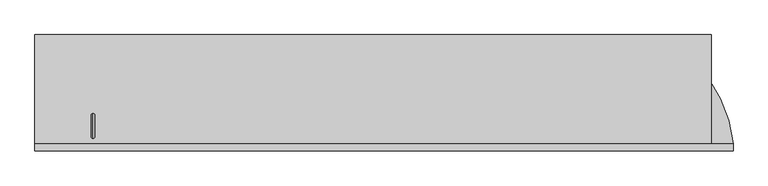
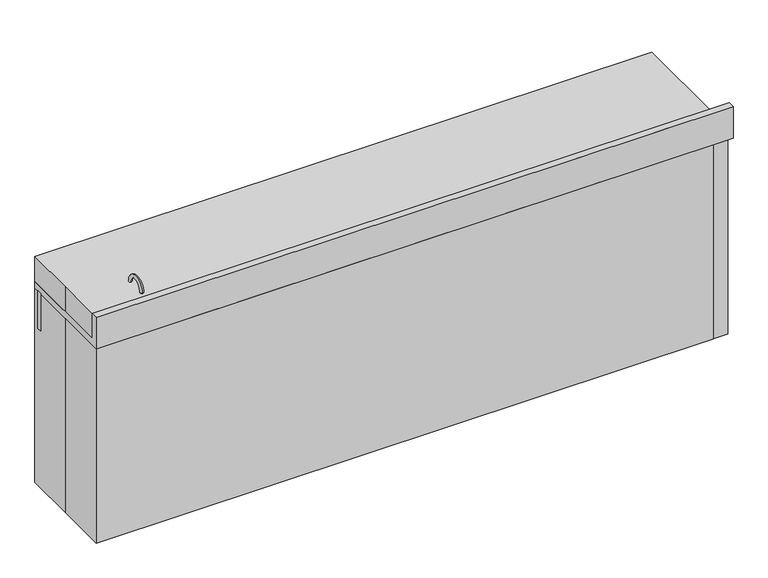
"""IFC4 building model written with IfcOpenShell, lengths in millimetres: proxy geometry, D0680 - Console, Accessory-Side, Dental Operatory-south sink-rounded : U0026 - Cabinet, Dental, Doctor's, Prosthodontic 2."""

import ifcopenshell
import ifcopenshell.guid

model = None  # the IFC model being written
_history = None  # IfcOwnerHistory: only IFC2X3 demands one
_inside = {}  # id of a spatial element -> (the spatial element, [elements in it])
_under = {}  # id of a project, library or spatial element -> (it, [spatial elements below it])
_declared = {}  # id of a project -> (the project, [libraries it declares])
_typed = {}  # id of a type object -> (the type object, [elements of that type])
_made_of = {}  # id of a material, layer set ... -> (it, [elements and type objects made of it])


def new_model(schema):
    """Start an empty IFC model of exactly this schema.

    Asked for "IFC4X3", IfcOpenShell would pick the latest addendum, in which some entities
    have other attributes; the version numbers below select the first issue.
    IFC2X3 requires an IfcOwnerHistory on every rooted entity: one is made here for all.
    """
    global model, _history
    if schema == "IFC4X3":
        model = ifcopenshell.file(schema_version=(4, 3, 0, 0))
    else:
        model = ifcopenshell.file(schema=schema)
    _inside.clear()
    _under.clear()
    _declared.clear()
    _typed.clear()
    _made_of.clear()
    _history = None
    if model.schema == "IFC2X3":
        org = make("IfcOrganization", Name="unknown")
        user = make(
            "IfcPersonAndOrganization",
            ThePerson=make("IfcPerson", FamilyName="unknown"),
            TheOrganization=org,
        )
        app = make(
            "IfcApplication",
            ApplicationDeveloper=org,
            Version="unknown",
            ApplicationFullName="unknown",
            ApplicationIdentifier="unknown",
        )
        _history = make(
            "IfcOwnerHistory",
            OwningUser=user,
            OwningApplication=app,
            ChangeAction="ADDED",
            CreationDate=0,
        )
    return model


def make(cls, **values):
    """One entity of the class cls with the attributes given. An attribute that is None is left unset."""
    return model.create_entity(
        cls, **{name: value for name, value in values.items() if value is not None}
    )


def rooted(cls, **values):
    """An entity with a GlobalId (a new one), such as an element, a storey or a relation."""
    return make(cls, GlobalId=ifcopenshell.guid.new(), OwnerHistory=_history, **values)


def si_unit(unit_type, name, prefix=None):
    """IfcSIUnit, for example si_unit("LENGTHUNIT", "METRE", prefix="MILLI")."""
    return make("IfcSIUnit", UnitType=unit_type, Prefix=prefix, Name=name)


def assignment(units):
    """IfcUnitAssignment: the units of a project."""
    return None if units is None else make("IfcUnitAssignment", Units=units)


def point(xyz):
    """IfcCartesianPoint."""
    return None if xyz is None else make("IfcCartesianPoint", Coordinates=xyz)


def direction(xyz):
    """IfcDirection."""
    return None if xyz is None else make("IfcDirection", DirectionRatios=xyz)


def frame(location, z_axis=None, x_axis=None):
    """IfcAxis2Placement3D, a coordinate frame: its origin and axes. An axis left out is left unset."""
    return make(
        "IfcAxis2Placement3D",
        Location=point(location),
        Axis=direction(z_axis),
        RefDirection=direction(x_axis),
    )


def frame_2d(location, x_axis=None):
    """IfcAxis2Placement2D, a coordinate frame in the plane: its origin and x axis."""
    return make(
        "IfcAxis2Placement2D", Location=point(location), RefDirection=direction(x_axis)
    )


def origin():
    """The frame at (0, 0, 0) with its axes left unset."""
    return frame((0.0, 0.0, 0.0))


def origin_with_axes():
    """The frame at (0, 0, 0) with the z axis (0, 0, 1) and the x axis (1, 0, 0) written out."""
    return frame((0.0, 0.0, 0.0), z_axis=(0.0, 0.0, 1.0), x_axis=(1.0, 0.0, 0.0))


def place(relative_to, where):
    """IfcLocalPlacement: puts the frame where relative to a parent placement (None: the world)."""
    return make(
        "IfcLocalPlacement", PlacementRelTo=relative_to, RelativePlacement=where
    )


def context(
    kind, dimensions, precision=None, world=None, true_north=None, identifier=None
):
    """IfcGeometricRepresentationContext, for example the 3D "Model" context."""
    return make(
        "IfcGeometricRepresentationContext",
        ContextIdentifier=identifier,
        ContextType=kind,
        CoordinateSpaceDimension=dimensions,
        Precision=precision,
        WorldCoordinateSystem=world,
        TrueNorth=true_north,
    )


def project(units=None, contexts=None):
    """IfcProject with its units and contexts."""
    return rooted(
        "IfcProject",
        Name="project",
        RepresentationContexts=contexts,
        UnitsInContext=assignment(units),
    )


def spatial(cls, under=None, at=None, **own):
    """A site, building, storey or space (cls), placed at a placement, below another one or the project."""
    s = rooted(cls, ObjectPlacement=at, **own)
    if under is not None:
        _under.setdefault(under.id(), (under, []))[1].append(s)
    return s


def polyline(points):
    """IfcPolyline through the points."""
    return make("IfcPolyline", Points=[point(p) for p in points])


def circle_curve(where, radius):
    """IfcCircle in the frame where."""
    return make("IfcCircle", Position=where, Radius=radius)


def ellipse_curve(where, semi_axis1, semi_axis2):
    """IfcEllipse in the frame where."""
    return make(
        "IfcEllipse", Position=where, SemiAxis1=semi_axis1, SemiAxis2=semi_axis2
    )


def trimmed(basis, trim1, trim2, sense, master):
    """IfcTrimmedCurve: the piece of a basis curve between two trims."""
    return make(
        "IfcTrimmedCurve",
        BasisCurve=basis,
        Trim1=trim1,
        Trim2=trim2,
        SenseAgreement=sense,
        MasterRepresentation=master,
    )


def segment(curve, same_sense, transition):
    """IfcCompositeCurveSegment."""
    return make(
        "IfcCompositeCurveSegment",
        Transition=transition,
        SameSense=same_sense,
        ParentCurve=curve,
    )


def composite_curve(segments, self_intersect=None):
    """IfcCompositeCurve: segments joined end to end."""
    return make("IfcCompositeCurve", Segments=segments, SelfIntersect=self_intersect)


def outline(outer, holes=None, kind="AREA"):
    """IfcArbitraryClosedProfileDef: a profile drawn as a closed curve; with holes, ...WithVoids."""
    if holes is None:
        return make("IfcArbitraryClosedProfileDef", ProfileType=kind, OuterCurve=outer)
    return make(
        "IfcArbitraryProfileDefWithVoids",
        ProfileType=kind,
        OuterCurve=outer,
        InnerCurves=holes,
    )


def extrude(swept, where, along, depth):
    """IfcExtrudedAreaSolid: the profile swept, set in the frame where, extruded along a direction by depth."""
    return make(
        "IfcExtrudedAreaSolid",
        SweptArea=swept,
        Position=where,
        ExtrudedDirection=direction(along),
        Depth=depth,
    )


def shape(context_of_items, identifier, shape_type, items):
    """IfcShapeRepresentation: the items that make up one representation, for example the "Body"."""
    return make(
        "IfcShapeRepresentation",
        ContextOfItems=context_of_items,
        RepresentationIdentifier=identifier,
        RepresentationType=shape_type,
        Items=items,
    )


def source(mapping_origin, context_of_items, identifier, shape_type, items):
    """IfcRepresentationMap: a shape defined once, which mapped items show again and again."""
    return make(
        "IfcRepresentationMap",
        MappingOrigin=mapping_origin,
        MappedRepresentation=shape(context_of_items, identifier, shape_type, items),
    )


def transform(
    local_origin,
    x_axis=None,
    y_axis=None,
    z_axis=None,
    scale=None,
    scale2=None,
    scale3=None,
    uniform=True,
):
    """IfcCartesianTransformationOperator3D, or its non-uniform kind. x_axis, y_axis, z_axis: its Axis1, 2, 3."""
    if uniform:
        return make(
            "IfcCartesianTransformationOperator3D",
            Axis1=direction(x_axis),
            Axis2=direction(y_axis),
            LocalOrigin=point(local_origin),
            Scale=scale,
            Axis3=direction(z_axis),
        )
    return make(
        "IfcCartesianTransformationOperator3DnonUniform",
        Axis1=direction(x_axis),
        Axis2=direction(y_axis),
        LocalOrigin=point(local_origin),
        Scale=scale,
        Axis3=direction(z_axis),
        Scale2=scale2,
        Scale3=scale3,
    )


def mapped(mapping_source, mapping_target):
    """IfcMappedItem: shows the shape of a source again, moved by a transform."""
    return make(
        "IfcMappedItem", MappingSource=mapping_source, MappingTarget=mapping_target
    )


def made_of(thing, what):
    """Note that an element or type object is made of a material, layer set ...; save() writes the relation."""
    if what is not None:
        _made_of.setdefault(what.id(), (what, []))[1].append(thing)
    return thing


def element(
    cls,
    number,
    at=None,
    inside=None,
    cuts=None,
    type_object=None,
    material=None,
    context=None,
    identifier="Body",
    shape_type=None,
    held_by="IfcProductDefinitionShape",
    body=None,
    shapes=None,
    **own,
):
    """One element of the class cls, such as IfcWall. Its Tag is "e" and its number.

    at: its placement. inside: the storey or other place that contains it. cuts: it is an
    opening in that element (IfcRelVoidsElement). A single representation is given by context,
    identifier, shape_type and body (its items); several are given by shapes. held_by: the class
    of the entity that holds the representations. save() writes the other relations.
    """
    e = rooted(cls, Tag="e%d" % number, ObjectPlacement=at, **own)
    if body is not None:
        shapes = [shape(context, identifier, shape_type, body)]
    if shapes is not None:
        e.Representation = make(held_by, Representations=shapes)
    if inside is not None:
        _inside.setdefault(inside.id(), (inside, []))[1].append(e)
    if cuts is not None:
        rooted(
            "IfcRelVoidsElement", RelatingBuildingElement=cuts, RelatedOpeningElement=e
        )
    if type_object is not None:
        _typed.setdefault(type_object.id(), (type_object, []))[1].append(e)
    return made_of(e, material)


def aggregate(whole, parts):
    """IfcRelAggregates: a whole, such as a stair, and the parts it consists of."""
    return rooted("IfcRelAggregates", RelatingObject=whole, RelatedObjects=parts)


def save(model, path):
    """Write the relations noted so far, then the file.

    IfcRelAggregates (storeys below a building ...), IfcRelContainedInSpatialStructure (elements
    in a storey), IfcRelDefinesByType, IfcRelAssociatesMaterial and IfcRelDeclares: one each for
    every whole, place, type object, material and project.
    """
    for whole, parts in _under.values():
        aggregate(whole, parts)
    for where, things in _inside.values():
        rooted(
            "IfcRelContainedInSpatialStructure",
            RelatedElements=things,
            RelatingStructure=where,
        )
    for kind, things in _typed.values():
        rooted("IfcRelDefinesByType", RelatedObjects=things, RelatingType=kind)
    for what, things in _made_of.values():
        rooted("IfcRelAssociatesMaterial", RelatedObjects=things, RelatingMaterial=what)
    for by, libraries in _declared.values():
        rooted("IfcRelDeclares", RelatingContext=by, RelatedDefinitions=libraries)
    model.write(path)


def plane_surface(at):
    """IfcPlane: the flat surface through the origin of the frame at, square to its z axis."""
    return make("IfcPlane", Position=at)


def cylinder_surface(at, radius):
    """IfcCylindricalSurface: all points at the distance radius from the z axis of the frame at."""
    return make("IfcCylindricalSurface", Position=at, Radius=radius)


def revolved_surface(curve, axis_point, axis_direction):
    """IfcSurfaceOfRevolution: the curve turned about the line through axis_point along axis_direction."""
    return make(
        "IfcSurfaceOfRevolution",
        SweptCurve=make("IfcArbitraryOpenProfileDef", ProfileType="CURVE", Curve=curve),
        AxisPosition=make("IfcAxis1Placement", Location=point(axis_point), Axis=direction(axis_direction)),
    )


def advanced_brep(points, edges, surfaces, faces):
    """IfcAdvancedBrep: a solid bounded by faces that lie on surfaces and meet in shared edges.

    An edge is (start, end): straight between two places in points (the first is 0);
    or (start, end, curve); or (start, end, curve, False) where it runs against its curve.
    A face is (place in surfaces, loops), or (place, loops, False) where it looks against
    its surface's normal. A loop lists edges by number (the first is 1), with a minus sign
    where the edge is run from its end to its start. The first loop is the outer one.
    """
    corners = [point(p) for p in points]
    vertices = [make("IfcVertexPoint", VertexGeometry=c) for c in corners]
    made = []
    for start, end, *more in edges:
        made.append(
            make(
                "IfcEdgeCurve",
                EdgeStart=vertices[start],
                EdgeEnd=vertices[end],
                EdgeGeometry=more[0] if more else make("IfcPolyline", Points=[corners[start], corners[end]]),
                SameSense=more[1] if len(more) > 1 else True,
            )
        )
    hull = []
    for where, loops, *sense in faces:
        bounds = []
        for j, loop in enumerate(loops):
            ring = [make("IfcOrientedEdge", EdgeElement=made[abs(k) - 1], Orientation=k > 0) for k in loop]
            bounds.append(
                make(
                    "IfcFaceOuterBound" if j == 0 else "IfcFaceBound",
                    Bound=make("IfcEdgeLoop", EdgeList=ring),
                    Orientation=True,
                )
            )
        hull.append(make("IfcAdvancedFace", Bounds=bounds, FaceSurface=surfaces[where], SameSense=sense[0] if sense else True))
    return make("IfcAdvancedBrep", Outer=make("IfcClosedShell", CfsFaces=hull))


def specialty_equipment_bc5c30ac(model_context):
    return source(origin(), model_context, "Body", "SolidModel", [
        advanced_brep(
        [(-1014.0443585, 165.0080446, 787.3899582), (-1014.0443585, 153.8955446, 787.3899582), (-1014.0443585, -128.6794554, 787.3899582), (-1014.0443585, -139.7919554, 787.3899582), (-1014.0443585, 152.3080446, 785.8024582), (-1014.0443585, -127.0919554, 785.8024582), (-1014.0443585, 152.3080446, 730.25), (-1014.0443585, -127.0919554, 730.25), (-1014.0443585, 101.5080446, 679.45), (-1014.0443585, 25.2053012, 679.45), (-1003.5461263, 12.6976148, 679.45), (-1014.0443585, 0.1899284, 679.45), (-1014.0443585, -76.2919554, 679.45), (-1028.9461263, 12.6976148, 679.45), (-1014.0443585, 158.6580446, 676.275), (-1014.0443585, 158.6580446, 784.0168572), (-1014.0443585, -133.4419554, 784.0168572), (-1014.0443585, -133.4419554, 676.275), (-1014.0443585, 165.0080446, 784.0168572), (-1014.0443585, -139.7919554, 784.0168572), (-1014.0443585, 0.1899284, 676.275), (-1003.5461263, 12.6976148, 676.275), (-1014.0443585, 25.2053012, 676.275), (-1028.9461263, 12.6976148, 676.275)],
        [
            (0, 1),
            (1, 2, circle_curve(frame((-1014.0443585, 12.6080446, 787.3899582), z_axis=(0.0, 0.0, -1.0), x_axis=(0.0, -1.0, 0.0)), 141.2875)),
            (2, 3),
            (3, 0, circle_curve(frame((-1014.0443585, 12.6080446, 787.3899582), z_axis=(0.0, 0.0, 1.0), x_axis=(0.0, -1.0, 0.0)), 152.4)),
            (2, 1, circle_curve(frame((-1014.0443585, 12.6080446, 787.3899582), z_axis=(0.0, 0.0, -1.0), x_axis=(0.0, -1.0, 0.0)), 141.2875)),
            (0, 3, circle_curve(frame((-1014.0443585, 12.6080446, 787.3899582), z_axis=(0.0, 0.0, 1.0), x_axis=(0.0, -1.0, 0.0)), 152.4)),
            (1, 4, circle_curve(frame((-1014.0443585, 153.8955446, 785.8024582), z_axis=(1.0, 0.0, 0.0), x_axis=(0.0, 1.0, 0.0)), 1.5875)),
            (4, 5, circle_curve(frame((-1014.0443585, 12.6080446, 785.8024582), z_axis=(0.0, 0.0, -1.0), x_axis=(0.0, -1.0, 0.0)), 139.7)),
            (5, 2, circle_curve(frame((-1014.0443585, -128.6794554, 785.8024582), z_axis=(1.0, 0.0, 0.0), x_axis=(0.0, -1.0, 0.0)), 1.5875)),
            (5, 4, circle_curve(frame((-1014.0443585, 12.6080446, 785.8024582), z_axis=(0.0, 0.0, -1.0), x_axis=(0.0, -1.0, 0.0)), 139.7)),
            (4, 6),
            (6, 7, circle_curve(frame((-1014.0443585, 12.6080446, 730.25), z_axis=(0.0, 0.0, -1.0), x_axis=(0.0, -1.0, 0.0)), 139.7)),
            (7, 5),
            (7, 6, circle_curve(frame((-1014.0443585, 12.6080446, 730.25), z_axis=(0.0, 0.0, -1.0), x_axis=(0.0, -1.0, 0.0)), 139.7)),
            (8, 9),
            (9, 10, circle_curve(frame((-1016.2461263, 12.6976148, 679.45), z_axis=(0.0, 0.0, -1.0), x_axis=(-1.0, 0.0, 0.0)), 12.7)),
            (10, 11, circle_curve(frame((-1016.2461263, 12.6976148, 679.45), z_axis=(0.0, 0.0, -1.0), x_axis=(-1.0, 0.0, 0.0)), 12.7)),
            (11, 12),
            (12, 8, circle_curve(frame((-1014.0443585, 12.6080446, 679.45), z_axis=(0.0, 0.0, 1.0), x_axis=(0.0, -1.0, 0.0)), 88.9)),
            (11, 13, circle_curve(frame((-1016.2461263, 12.6976148, 679.45), z_axis=(0.0, 0.0, -1.0), x_axis=(-1.0, 0.0, 0.0)), 12.7)),
            (13, 9, circle_curve(frame((-1016.2461263, 12.6976148, 679.45), z_axis=(0.0, 0.0, -1.0), x_axis=(-1.0, 0.0, 0.0)), 12.7)),
            (8, 12, circle_curve(frame((-1014.0443585, 12.6080446, 679.45), z_axis=(0.0, 0.0, 1.0), x_axis=(0.0, -1.0, 0.0)), 88.9)),
            (14, 15),
            (15, 16, circle_curve(frame((-1014.0443585, 12.6080446, 784.0168572), z_axis=(0.0, 0.0, -1.0), x_axis=(0.0, -1.0, 0.0)), 146.05)),
            (16, 17),
            (17, 14, circle_curve(frame((-1014.0443585, 12.6080446, 676.275), z_axis=(0.0, 0.0, 1.0), x_axis=(0.0, -1.0, 0.0)), 146.05)),
            (16, 15, circle_curve(frame((-1014.0443585, 12.6080446, 784.0168572), z_axis=(0.0, 0.0, -1.0), x_axis=(0.0, -1.0, 0.0)), 146.05)),
            (14, 17, circle_curve(frame((-1014.0443585, 12.6080446, 676.275), z_axis=(0.0, 0.0, 1.0), x_axis=(0.0, -1.0, 0.0)), 146.05)),
            (15, 18),
            (18, 19, circle_curve(frame((-1014.0443585, 12.6080446, 784.0168572), z_axis=(0.0, 0.0, -1.0), x_axis=(0.0, -1.0, 0.0)), 152.4)),
            (19, 16),
            (19, 18, circle_curve(frame((-1014.0443585, 12.6080446, 784.0168572), z_axis=(0.0, 0.0, -1.0), x_axis=(0.0, -1.0, 0.0)), 152.4)),
            (3, 19),
            (18, 0),
            (17, 20),
            (20, 21, circle_curve(frame((-1016.2461263, 12.6976148, 676.275), z_axis=(0.0, 0.0, 1.0), x_axis=(-1.0, 0.0, 0.0)), 12.7)),
            (21, 22, circle_curve(frame((-1016.2461263, 12.6976148, 676.275), z_axis=(0.0, 0.0, 1.0), x_axis=(-1.0, 0.0, 0.0)), 12.7)),
            (22, 14),
            (22, 23, circle_curve(frame((-1016.2461263, 12.6976148, 676.275), z_axis=(0.0, 0.0, 1.0), x_axis=(-1.0, 0.0, 0.0)), 12.7)),
            (23, 20, circle_curve(frame((-1016.2461263, 12.6976148, 676.275), z_axis=(0.0, 0.0, 1.0), x_axis=(-1.0, 0.0, 0.0)), 12.7)),
            (6, 8, circle_curve(frame((-1014.0443585, 101.5080446, 730.25), z_axis=(-1.0, 0.0, 0.0), x_axis=(0.0, 1.0, 0.0)), 50.8)),
            (12, 7, circle_curve(frame((-1014.0443585, -76.2919554, 730.25), z_axis=(-1.0, 0.0, 0.0), x_axis=(0.0, -1.0, 0.0)), 50.8)),
            (21, 10),
            (13, 23),
        ],
        [
            plane_surface(frame((-1014.0443585, 12.6080446, 787.3899582), z_axis=(0.0, 0.0, 1.0), x_axis=(0.0, -1.0, 0.0))),
            revolved_surface(trimmed(ellipse_curve(frame((-1014.0443585, -128.6794554, 785.8024582), z_axis=(1.0, 0.0, 0.0), x_axis=(0.0, -1.0, 0.0)), 1.5875, 1.5875), [point((-1014.0443585, -127.0919554, 785.8024582))], [point((-1014.0443585, -128.6794554, 787.3899582))], True, "CARTESIAN"), (-1014.0443585, 12.6080446, 787.4), (0.0, 0.0, -1.0)),
            revolved_surface(polyline([(-1014.0443585, -127.09195539999999, 730.25), (-1014.0443585, -127.09195539999999, 785.8024582)]), (-1014.0443585, 12.6080446, 787.4), (0.0, 0.0, -1.0)),
            plane_surface(frame((-1014.0443585, 12.6080446, 679.45), z_axis=(0.0, 0.0, 1.0), x_axis=(0.0, -1.0, 0.0))),
            cylinder_surface(frame((-1014.0443585, 12.6080446, 787.4), z_axis=(0.0, 0.0, -1.0), x_axis=(0.0, -1.0, 0.0)), 146.05),
            plane_surface(frame((-1014.0443585, 12.6080446, 784.0168572), z_axis=(0.0, 0.0, -1.0), x_axis=(0.0, -1.0, 0.0))),
            cylinder_surface(frame((-1014.0443585, 12.6080446, 787.4), z_axis=(0.0, 0.0, -1.0), x_axis=(0.0, -1.0, 0.0)), 152.4),
            plane_surface(frame((-1014.0443585, 12.6080446, 676.275), z_axis=(0.0, 0.0, -1.0), x_axis=(0.0, -1.0, 0.0))),
            revolved_surface(trimmed(ellipse_curve(frame((-1014.0443585, -76.2919554, 730.25), z_axis=(-1.0, 0.0, 0.0), x_axis=(0.0, -1.0, 0.0)), 50.8, 50.8), [point((-1014.0443585, -76.2919554, 679.45))], [point((-1014.0443585, -127.0919554, 730.25))], True, "CARTESIAN"), (-1014.0443585, 12.6080446, 787.4), (0.0, 0.0, -1.0)),
            revolved_surface(polyline([(-1028.9461263, 12.6976148, 679.45), (-1028.9461263, 12.6976148, 676.275)]), (-1016.2461263, 12.6976148, 673.1), (0.0, 0.0, 1.0)),
        ],
        [
            (0, [[1, 2, 3, 4]]),
            (0, [[5, -1, 6, -3]]),
            (1, [[7, 8, 9, -2]]),
            (1, [[-9, 10, -7, -5]]),
            (2, [[11, 12, 13, -8]]),
            (2, [[-13, 14, -11, -10]]),
            (3, [[15, 16, 17, 18, 19]]),
            (3, [[-18, 20, 21, -15, 22]]),
            (4, [[23, 24, 25, 26]]),
            (4, [[27, -23, 28, -25]]),
            (5, [[29, 30, 31, -24]]),
            (5, [[-31, 32, -29, -27]]),
            (6, [[33, -30, 34, -4]]),
            (6, [[-34, -32, -33, -6]]),
            (7, [[35, 36, 37, 38, -26]]),
            (7, [[-38, 39, 40, -35, -28]]),
            (8, [[41, -19, 42, -12]]),
            (8, [[-42, -22, -41, -14]]),
            (9, [[-39, -37, 43, -16, -21, 44]]),
            (9, [[-20, -17, -43, -36, -40, -44]]),
        ],
    ),
        extrude(outline(polyline([(-1219.2, 184.15), (-850.9, 184.15), (-850.9, 165.1), (-1219.2, 165.1), (-1219.2, 184.15)])), frame((0.0, 0.0, 635.0), z_axis=(0.0, 0.0, 1.0), x_axis=(1.0, 0.0, 0.0)), (0.0, 0.0, 1.0), 152.4),
        extrude(outline(polyline([(184.15, 101.6), (184.15, 787.2846899), (193.675, 787.2846899), (193.675, 774.4822891), (203.2, 774.4822891), (203.2, 101.6), (184.15, 101.6)])), frame((584.2, 0.0, 0.0), z_axis=(1.0, 0.0, 0.0), x_axis=(0.0, 1.0, 0.0)), (0.0, 0.0, 1.0), 355.6),
        extrude(outline(polyline([(184.15, 101.6), (184.15, 787.4), (193.675, 787.4), (193.675, 774.7), (203.2, 774.7), (203.2, 101.6), (184.15, 101.6)])), frame((228.6, 0.0, 0.0), z_axis=(1.0, 0.0, 0.0), x_axis=(0.0, 1.0, 0.0)), (0.0, 0.0, 1.0), 355.6),
        extrude(outline(polyline([(184.15, 101.6), (184.15, 787.4), (193.675, 787.4), (193.675, 774.7), (203.2, 774.7), (203.2, 101.6), (184.15, 101.6)])), frame((-127.0, 0.0, 0.0), z_axis=(1.0, 0.0, 0.0), x_axis=(0.0, 1.0, 0.0)), (0.0, 0.0, 1.0), 355.6),
        extrude(outline(polyline([(193.675, 774.7), (203.2, 774.7), (203.2, 635.0), (184.15, 635.0), (184.15, 787.4), (193.675, 787.4), (193.675, 774.7)])), frame((-482.6, 0.0, 0.0), z_axis=(1.0, 0.0, 0.0), x_axis=(0.0, 1.0, 0.0)), (0.0, 0.0, 1.0), 355.6),
        extrude(outline(polyline([(193.675, 622.9156171), (203.2, 622.9156171), (203.2, 508.0524006), (184.15, 508.0524006), (184.15, 635.0), (193.675, 635.0), (193.675, 622.9156171)])), frame((-482.6, 0.0, 0.0), z_axis=(1.0, 0.0, 0.0), x_axis=(0.0, 1.0, 0.0)), (0.0, 0.0, 1.0), 355.6),
        extrude(outline(polyline([(193.675, 495.2120809), (203.2, 495.2120809), (203.2, 101.6), (184.15, 101.6), (184.15, 508.0517033), (193.675, 508.0517033), (193.675, 495.2120809)])), frame((-482.6, 0.0, 0.0), z_axis=(1.0, 0.0, 0.0), x_axis=(0.0, 1.0, 0.0)), (0.0, 0.0, 1.0), 355.6),
        extrude(outline(composite_curve([segment(trimmed(circle_curve(frame_2d((-1053.7479232, -156.0133962)), 12.7), [point((-1041.0479232, -156.0133962))], [point((-1066.4479232, -156.0133962))], False, "CARTESIAN"), True, "CONTINUOUS"), segment(trimmed(circle_curve(frame_2d((-1053.7479232, -156.0133962)), 12.7), [point((-1066.4479232, -156.0133962))], [point((-1041.0479232, -156.0133962))], False, "CARTESIAN"), True, "CONTINUOUS")], self_intersect=False)), frame((0.0, 0.0, 812.8), z_axis=(0.0, 0.0, 1.0), x_axis=(1.0, 0.0, 0.0)), (0.0, 0.0, 1.0), 31.75),
        extrude(outline(composite_curve([segment(trimmed(circle_curve(frame_2d((-980.5384765, -156.0133962)), 12.7), [point((-967.8384765, -156.0133962))], [point((-993.2384765, -156.0133962))], False, "CARTESIAN"), True, "CONTINUOUS"), segment(trimmed(circle_curve(frame_2d((-980.5384765, -156.0133962)), 12.7), [point((-993.2384765, -156.0133962))], [point((-967.8384765, -156.0133962))], False, "CARTESIAN"), True, "CONTINUOUS")], self_intersect=False)), frame((0.0, 0.0, 812.8), z_axis=(0.0, 0.0, 1.0), x_axis=(1.0, 0.0, 0.0)), (0.0, 0.0, 1.0), 31.75),
        advanced_brep(
        [(-1016.415785, -148.0147812, 812.8), (-1016.415785, -160.7147812, 812.8), (-1016.415785, -148.0147812, 914.4), (-1016.415785, -160.7147812, 914.4), (-1016.415785, -84.5147812, 914.4), (-1016.415785, -71.8147812, 914.4)],
        [
            (0, 1, circle_curve(frame((-1016.415785, -154.3647812, 812.8), z_axis=(0.0, 0.0, -1.0), x_axis=(0.0, -1.0, 0.0)), 6.35)),
            (1, 0, circle_curve(frame((-1016.415785, -154.3647812, 812.8), z_axis=(0.0, 0.0, -1.0), x_axis=(0.0, -1.0, 0.0)), 6.35)),
            (0, 2),
            (2, 3, circle_curve(frame((-1016.415785, -154.3647812, 914.4), z_axis=(0.0, 0.0, -1.0), x_axis=(0.0, -1.0, 0.0)), 6.35)),
            (3, 1),
            (3, 2, circle_curve(frame((-1016.415785, -154.3647812, 914.4), z_axis=(0.0, 0.0, -1.0), x_axis=(0.0, -1.0, 0.0)), 6.35)),
            (4, 5, circle_curve(frame((-1016.415785, -78.1647812, 914.4), z_axis=(0.0, 0.0, -1.0), x_axis=(0.0, 1.0, 0.0)), 6.35)),
            (5, 4, circle_curve(frame((-1016.415785, -78.1647812, 914.4), z_axis=(0.0, 0.0, -1.0), x_axis=(0.0, 1.0, 0.0)), 6.35)),
            (5, 3, circle_curve(frame((-1016.415785, -116.2647812, 914.4), z_axis=(1.0, 0.0, 0.0), x_axis=(0.0, -1.0, 0.0)), 44.45)),
            (2, 4, circle_curve(frame((-1016.415785, -116.2647812, 914.4), z_axis=(-1.0, 0.0, 0.0), x_axis=(0.0, -1.0, 0.0)), 31.75)),
        ],
        [
            plane_surface(frame((-1104.9, -154.3647812, 812.8), z_axis=(0.0, 0.0, -1.0), x_axis=(-1.0, 0.0, 0.0))),
            cylinder_surface(frame((-1016.415785, -154.3647812, 812.8), z_axis=(0.0, 0.0, -1.0), x_axis=(0.0, -1.0, 0.0)), 6.35),
            plane_surface(frame((-1104.9, -78.1647812, 914.4), z_axis=(0.0, 0.0, -1.0), x_axis=(-1.0, 0.0, 0.0))),
            revolved_surface(trimmed(ellipse_curve(frame((-1016.415785, -154.3647812, 914.4), z_axis=(0.0, 0.0, 1.0), x_axis=(0.0, -1.0, 0.0)), 6.35, 6.35), [point((-1016.415785, -160.7147812, 914.4))], [point((-1016.415785, -148.0147812, 914.4))], True, "CARTESIAN"), (-1104.9, -116.2647812, 914.4), (1.0, 0.0, 0.0)),
            revolved_surface(trimmed(ellipse_curve(frame((-1016.415785, -154.3647812, 914.4), z_axis=(0.0, 0.0, 1.0), x_axis=(0.0, -1.0, 0.0)), 6.35, 6.35), [point((-1016.415785, -148.0147812, 914.4))], [point((-1016.415785, -160.7147812, 914.4))], True, "CARTESIAN"), (-1104.9, -116.2647812, 914.4), (1.0, 0.0, 0.0)),
        ],
        [
            (0, [[1, 2]]),
            (1, [[3, 4, 5, -1]]),
            (1, [[-5, 6, -3, -2]]),
            (2, [[7, 8]]),
            (3, [[-8, 9, -4, 10]]),
            (4, [[-7, -10, -6, -9]]),
        ],
    ),
        extrude(outline(polyline([(193.675, 774.7), (203.2, 774.7), (203.2, 635.0), (184.15, 635.0), (184.15, 787.4), (193.675, 787.4), (193.675, 774.7)])), frame((-838.2, 0.0, 0.0), z_axis=(1.0, 0.0, 0.0), x_axis=(0.0, 1.0, 0.0)), (0.0, 0.0, 1.0), 355.6),
        extrude(outline(polyline([(193.675, 622.9156171), (203.2, 622.9156171), (203.2, 508.0), (184.15, 508.0), (184.15, 635.0), (193.675, 635.0), (193.675, 622.9156171)])), frame((-838.2, 0.0, 0.0), z_axis=(1.0, 0.0, 0.0), x_axis=(0.0, 1.0, 0.0)), (0.0, 0.0, 1.0), 355.6),
        extrude(outline(polyline([(193.675, 495.3), (203.2, 495.3), (203.2, 406.4), (184.15, 406.4), (184.15, 508.0), (193.675, 508.0), (193.675, 495.3)])), frame((-838.2, 0.0, 0.0), z_axis=(1.0, 0.0, 0.0), x_axis=(0.0, 1.0, 0.0)), (0.0, 0.0, 1.0), 355.6),
        extrude(outline(polyline([(193.675, 393.7), (203.2, 393.7), (203.2, 304.8), (184.15, 304.8), (184.15, 406.4), (193.675, 406.4), (193.675, 393.7)])), frame((-838.2, 0.0, 0.0), z_axis=(1.0, 0.0, 0.0), x_axis=(0.0, 1.0, 0.0)), (0.0, 0.0, 1.0), 355.6),
        extrude(outline(polyline([(193.675, 292.1), (203.2, 292.1), (203.2, 101.6), (184.15, 101.6), (184.15, 304.8), (193.675, 304.8), (193.675, 292.1)])), frame((-838.2, 0.0, 0.0), z_axis=(1.0, 0.0, 0.0), x_axis=(0.0, 1.0, 0.0)), (0.0, 0.0, 1.0), 355.6),
        advanced_brep(
        [(-1219.2, -177.8, 914.4), (-1219.2, -177.8, 812.8), (-1219.2, 203.2, 812.8), (-1219.2, 203.2, 787.4), (-1219.2, -203.2, 787.4), (-1219.2, -203.2, 914.4), (1219.2, -177.8, 914.4), (1219.2, -177.8, 863.6), (1219.2, -177.8, 812.8), (939.8, 203.2, 812.8), (-874.2071906, 12.5959993, 812.8), (-1153.6071906, 12.5959993, 812.8), (939.8, 203.2, 787.4), (1219.2, -177.8, 787.4), (1219.2, -203.2, 787.4), (-1153.6071906, 12.5959993, 787.4), (-874.2071906, 12.5959993, 787.4), (1219.2, -203.2, 914.4)],
        [
            (0, 1),
            (1, 2),
            (2, 3),
            (3, 4),
            (4, 5),
            (5, 0),
            (0, 6),
            (6, 7),
            (7, 8),
            (8, 1),
            (8, 9, circle_curve(frame((763.8405952, -218.7835635, 812.8), z_axis=(0.0, 0.0, 1.0), x_axis=(1.0, 0.0, 0.0)), 457.2)),
            (9, 2),
            (10, 11, circle_curve(frame((-1013.9071906, 12.5959993, 812.8), z_axis=(0.0, 0.0, -1.0), x_axis=(-1.0, 0.0, 0.0)), 139.7)),
            (11, 10, circle_curve(frame((-1013.9071906, 12.5959993, 812.8), z_axis=(0.0, 0.0, -1.0), x_axis=(-1.0, 0.0, 0.0)), 139.7)),
            (9, 12),
            (12, 3),
            (12, 13, circle_curve(frame((763.8405952, -218.7835635, 787.4), z_axis=(0.0, 0.0, -1.0), x_axis=(1.0, 0.0, 0.0)), 457.2)),
            (13, 14),
            (14, 4),
            (15, 16, circle_curve(frame((-1013.9071906, 12.5959993, 787.4), z_axis=(0.0, 0.0, 1.0), x_axis=(-1.0, 0.0, 0.0)), 139.7)),
            (16, 15, circle_curve(frame((-1013.9071906, 12.5959993, 787.4), z_axis=(0.0, 0.0, 1.0), x_axis=(-1.0, 0.0, 0.0)), 139.7)),
            (17, 5),
            (14, 17),
            (17, 6),
            (16, 10),
            (11, 15),
            (13, 8),
        ],
        [
            plane_surface(frame((-1219.2, -177.8, 812.8), z_axis=(-1.0, 0.0, 0.0), x_axis=(0.0, 0.0, 1.0))),
            plane_surface(frame((1219.2, -177.8, 914.4), z_axis=(0.0, 1.0, 0.0), x_axis=(-1.0, 0.0, 0.0))),
            plane_surface(frame((1219.2, -177.8, 812.8), z_axis=(0.0, 0.0, 1.0), x_axis=(-1.0, 0.0, 0.0))),
            plane_surface(frame((1219.2, 203.2, 812.8), z_axis=(0.0, 1.0, 0.0), x_axis=(-1.0, 0.0, 0.0))),
            plane_surface(frame((1219.2, 203.2, 787.4), z_axis=(0.0, 0.0, -1.0), x_axis=(-1.0, 0.0, 0.0))),
            plane_surface(frame((1219.2, -203.2, 787.4), z_axis=(0.0, -1.0, 0.0), x_axis=(-1.0, 0.0, 0.0))),
            plane_surface(frame((1219.2, -203.2, 914.4), z_axis=(0.0, 0.0, 1.0), x_axis=(-1.0, 0.0, 0.0))),
            revolved_surface(polyline([(-1153.6071906, 12.5959993, 812.8), (-1153.6071906, 12.5959993, 787.4)]), (-1013.9071906, 12.5959993, 768.35), (0.0, 0.0, 1.0)),
            plane_surface(frame((1219.2, -177.8, 812.8), z_axis=(1.0, 0.0, 0.0), x_axis=(0.0, 0.0, -1.0))),
            cylinder_surface(frame((763.8405952, -218.7835635, 736.6), z_axis=(0.0, 0.0, -1.0), x_axis=(1.0, 0.0, 0.0)), 457.2),
        ],
        [
            (0, [[1, 2, 3, 4, 5, 6]]),
            (1, [[7, 8, 9, 10, -1]]),
            (2, [[-10, 11, 12, -2], [13, 14]]),
            (3, [[-12, 15, 16, -3]]),
            (4, [[-16, 17, 18, 19, -4], [20, 21]]),
            (5, [[22, -5, -19, 23]]),
            (6, [[-7, -6, -22, 24]]),
            (7, [[-21, 25, -14, 26]]),
            (7, [[-13, -25, -20, -26]]),
            (8, [[-18, 27, -9, -8, -24, -23]]),
            (9, [[-17, -15, -11, -27]]),
        ],
    ),
        extrude(outline(polyline([(-1219.2, -203.2), (-1219.2, 0.0), (-1219.2, 203.2), (1143.0, 203.2), (1143.0, -203.2), (-1219.2, -203.2)])), origin_with_axes(), (0.0, 0.0, 1.0), 914.4),
        extrude(outline(polyline([(-184.15, 785.890324), (184.15, 785.890324), (184.15, 101.6), (165.1, 101.6), (165.1, 0.0), (-184.15, 0.0), (-184.15, 785.890324)])), frame((939.8, 0.0, 0.0), z_axis=(1.0, 0.0, 0.0), x_axis=(0.0, 1.0, 0.0)), (0.0, 0.0, 1.0), 12.7),
        extrude(outline(polyline([(1199.3554733, -184.15), (1199.3554733, -203.2), (-850.9, -203.2), (-850.9, -184.15), (1199.3554733, -184.15)])), origin_with_axes(), (0.0, 0.0, 1.0), 787.6898809),
        extrude(outline(polyline([(-117.475, -184.15), (-136.525, -184.15), (-136.525, 184.15), (-117.475, 184.15), (-117.475, -184.15)])), frame((0.0, 0.0, 120.7166954), z_axis=(0.0, 0.0, 1.0), x_axis=(1.0, 0.0, 0.0)), (0.0, 0.0, 1.0), 653.9833046),
        extrude(outline(polyline([(-184.15, 787.4), (184.15, 787.4), (184.15, 101.6), (165.1, 101.6), (165.1, 0.0), (-184.15, 0.0), (-184.15, 787.4)])), frame((-850.9, 0.0, 0.0), z_axis=(1.0, 0.0, 0.0), x_axis=(0.0, 1.0, 0.0)), (0.0, 0.0, 1.0), 12.7),
        extrude(outline(polyline([(-473.075, -184.15), (-492.125, -184.15), (-492.125, 184.15), (-473.075, 184.15), (-473.075, -184.15)])), frame((0.0, 0.0, 120.7166954), z_axis=(0.0, 0.0, 1.0), x_axis=(1.0, 0.0, 0.0)), (0.0, 0.0, 1.0), 666.6833046),
        extrude(outline(polyline([(952.5, 184.15), (952.5, 165.1), (-850.9, 165.1), (-850.9, 184.15), (952.5, 184.15)])), origin_with_axes(), (0.0, 0.0, 1.0), 101.6),
        extrude(outline(polyline([(-838.2, -184.15), (-838.2, 184.15), (939.8, 184.15), (939.8, -184.15), (-838.2, -184.15)])), frame((0.0, 0.0, 101.6), z_axis=(0.0, 0.0, 1.0), x_axis=(1.0, 0.0, 0.0)), (0.0, 0.0, 1.0), 19.1166954),
    ])


if __name__ == "__main__":
    model = new_model("IFC4")
    model_context = context("Model", 3, world=origin())
    ifc_project = project(units=[si_unit("LENGTHUNIT", "METRE", prefix="MILLI")], contexts=[model_context])
    site = spatial("IfcSite", under=ifc_project)
    building = spatial("IfcBuilding", under=site)
    placement = place(None, origin())
    specialty_equipment_shape = specialty_equipment_bc5c30ac(model_context)
    element("IfcBuildingElementProxy", 1, Name="D0680 - Console, Accessory-Side, Dental Operatory-south sink-rounded : U0026 - Cabinet, Dental, Doctor's, Prosthodontic 2", ObjectType="D0680 - Console, Accessory-Side, Dental Operatory-south sink-rounded : U0026 - Cabinet, Dental, Doctor's, Prosthodontic 2", at=placement, inside=building, context=model_context, shape_type="MappedRepresentation", body=[
        mapped(specialty_equipment_shape, transform((0.0, 0.0, 0.0), x_axis=(1.0, 0.0, 0.0), y_axis=(0.0, 1.0, 0.0), z_axis=(0.0, 0.0, 1.0))),
    ])
    save(model, "model.ifc")

# Revit data of these elements
# Type "D0680 - Console, Accessory-Side, Dental Operatory-south sink-rounded : U0026 - Cabinet, Dental, Doctor's, Prosthodontic 2"
#   Watts2 = "0"
#   Watts1 = "120"
#   Unit_Issue = "EA"
#   UTIL_6_Misc = "-"
#   UTIL_5_NonMedGas = "-"
#   UTIL_4_MiscGas = "-"
#   UTIL_3_MedGas = "-"
#   UTIL_2_Elec = "A"
#   UTIL_1_WaterDrain = "D"
#   Nomenclature = "Console, Accessory/Side, Dental Operatory"
#   NSN = "6520"
#   Location [instance default] = ""
#   JSN = "D0680"
#   Fund_Source_VA = "-"
#   Fund_Source_Navy = "-"
#   Fund_Source_Army = "-"
#   Fund_Source_AF = "-"
#   ELEC_Volts2 = "0"
#   ELEC_Volts1 = "120"
#   ELEC_Phase2 = "0"
#   ELEC_Phase1 = "1"
#   ELEC_HertzSwitch = "0"
#   ELEC_HertzDependent = "-1"
#   ELEC_Hertz = "60"
#   ELEC_Amps2 = "0"
#   ELEC_Amps1 = "1"
#   DetailDescription = "An accessory or side console/cabinet approximately 60\" W x24\"D x 32\"H for use in a single chair dental operatory. The console may be a left or a right unit used for the dentist or the assistant depending configuration of the operatory. The unit may contain a sink component with waste drop, a round SS sink with faucet and soap dispenser, a solid surface counter top, a drawer storage module with writing surface and equipment drawers, a double door component with swing out shelves and a glove dispenser. Various combinations are available as well as different widths. Configuration of the unit, including whether the unit is right or left, to be determined at time of purchase."
#   CAT_VA = "A"
#   CAT_Navy = "A"
#   CAT_IHS = "-"
#   CAT_Army = "A"
#   CAT_AF = "A"
#   BTUperhour = "0"
#   Weight_IP = 0
#   DIM_Width_IP = 5' - 5"
#   DIM_Height_IP = 2' - 8"
#   DIM_Depth_IP = 2' - 5"
#   Shelf Panel Material = none
#   Assembly Code = ""
# Element 1 (IfcBuildingElementProxy, "D0680 - Console, Accessory-Side, Dental Operatory-south sink-rounded : U0026 - Cabinet, Dental, Doctor's, Prosthodontic 2")
#   Materials on its faces: "CabinetFinish", "CounterTopFinish", "EquipSpace"
# Materials
#   "CabinetFinish": class "Unassigned", colour RGB 245 239 218, transparency 0
#   "CounterTopFinish": class "Unassigned", colour RGB 139 121 96, transparency 0
#   "EquipSpace": class "Unassigned", colour RGB 221 217 195, transparency 0.5
